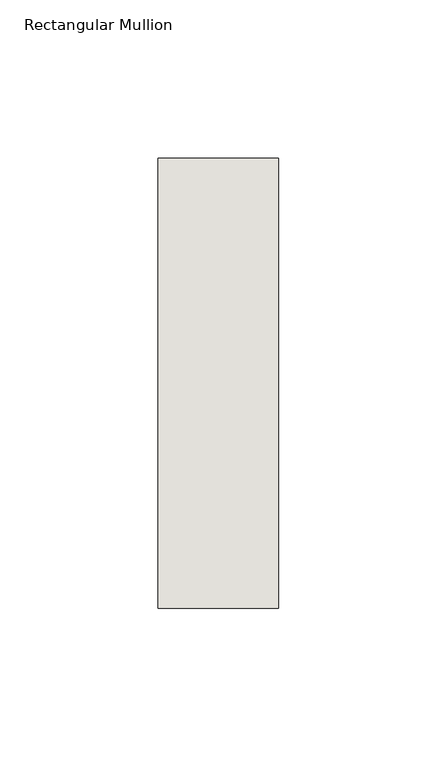
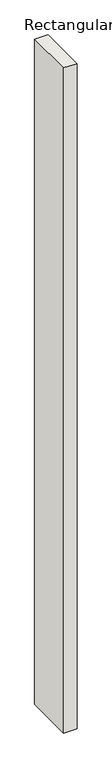
"""IFC4 building model written with IfcOpenShell, lengths in millimetres: wall geometry, Rectangular Mullion : NLRS_21_CWM_hsb-regel 38x142_gen_rsf."""

import ifcopenshell
import ifcopenshell.guid

model = None  # the IFC model being written
_history = None  # IfcOwnerHistory: only IFC2X3 demands one
_inside = {}  # id of a spatial element -> (the spatial element, [elements in it])
_under = {}  # id of a project, library or spatial element -> (it, [spatial elements below it])
_declared = {}  # id of a project -> (the project, [libraries it declares])
_typed = {}  # id of a type object -> (the type object, [elements of that type])
_made_of = {}  # id of a material, layer set ... -> (it, [elements and type objects made of it])


def new_model(schema):
    """Start an empty IFC model of exactly this schema.

    Asked for "IFC4X3", IfcOpenShell would pick the latest addendum, in which some entities
    have other attributes; the version numbers below select the first issue.
    IFC2X3 requires an IfcOwnerHistory on every rooted entity: one is made here for all.
    """
    global model, _history
    if schema == "IFC4X3":
        model = ifcopenshell.file(schema_version=(4, 3, 0, 0))
    else:
        model = ifcopenshell.file(schema=schema)
    _inside.clear()
    _under.clear()
    _declared.clear()
    _typed.clear()
    _made_of.clear()
    _history = None
    if model.schema == "IFC2X3":
        org = make("IfcOrganization", Name="unknown")
        user = make(
            "IfcPersonAndOrganization",
            ThePerson=make("IfcPerson", FamilyName="unknown"),
            TheOrganization=org,
        )
        app = make(
            "IfcApplication",
            ApplicationDeveloper=org,
            Version="unknown",
            ApplicationFullName="unknown",
            ApplicationIdentifier="unknown",
        )
        _history = make(
            "IfcOwnerHistory",
            OwningUser=user,
            OwningApplication=app,
            ChangeAction="ADDED",
            CreationDate=0,
        )
    return model


def make(cls, **values):
    """One entity of the class cls with the attributes given. An attribute that is None is left unset."""
    return model.create_entity(
        cls, **{name: value for name, value in values.items() if value is not None}
    )


def rooted(cls, **values):
    """An entity with a GlobalId (a new one), such as an element, a storey or a relation."""
    return make(cls, GlobalId=ifcopenshell.guid.new(), OwnerHistory=_history, **values)


def si_unit(unit_type, name, prefix=None):
    """IfcSIUnit, for example si_unit("LENGTHUNIT", "METRE", prefix="MILLI")."""
    return make("IfcSIUnit", UnitType=unit_type, Prefix=prefix, Name=name)


def assignment(units):
    """IfcUnitAssignment: the units of a project."""
    return None if units is None else make("IfcUnitAssignment", Units=units)


def point(xyz):
    """IfcCartesianPoint."""
    return None if xyz is None else make("IfcCartesianPoint", Coordinates=xyz)


def direction(xyz):
    """IfcDirection."""
    return None if xyz is None else make("IfcDirection", DirectionRatios=xyz)


def frame(location, z_axis=None, x_axis=None):
    """IfcAxis2Placement3D, a coordinate frame: its origin and axes. An axis left out is left unset."""
    return make(
        "IfcAxis2Placement3D",
        Location=point(location),
        Axis=direction(z_axis),
        RefDirection=direction(x_axis),
    )


def origin():
    """The frame at (0, 0, 0) with its axes left unset."""
    return frame((0.0, 0.0, 0.0))


def place(relative_to, where):
    """IfcLocalPlacement: puts the frame where relative to a parent placement (None: the world)."""
    return make(
        "IfcLocalPlacement", PlacementRelTo=relative_to, RelativePlacement=where
    )


def context(
    kind, dimensions, precision=None, world=None, true_north=None, identifier=None
):
    """IfcGeometricRepresentationContext, for example the 3D "Model" context."""
    return make(
        "IfcGeometricRepresentationContext",
        ContextIdentifier=identifier,
        ContextType=kind,
        CoordinateSpaceDimension=dimensions,
        Precision=precision,
        WorldCoordinateSystem=world,
        TrueNorth=true_north,
    )


def project(units=None, contexts=None):
    """IfcProject with its units and contexts."""
    return rooted(
        "IfcProject",
        Name="project",
        RepresentationContexts=contexts,
        UnitsInContext=assignment(units),
    )


def spatial(cls, under=None, at=None, **own):
    """A site, building, storey or space (cls), placed at a placement, below another one or the project."""
    s = rooted(cls, ObjectPlacement=at, **own)
    if under is not None:
        _under.setdefault(under.id(), (under, []))[1].append(s)
    return s


def polyline(points):
    """IfcPolyline through the points."""
    return make("IfcPolyline", Points=[point(p) for p in points])


def outline(outer, holes=None, kind="AREA"):
    """IfcArbitraryClosedProfileDef: a profile drawn as a closed curve; with holes, ...WithVoids."""
    if holes is None:
        return make("IfcArbitraryClosedProfileDef", ProfileType=kind, OuterCurve=outer)
    return make(
        "IfcArbitraryProfileDefWithVoids",
        ProfileType=kind,
        OuterCurve=outer,
        InnerCurves=holes,
    )


def extrude(swept, where, along, depth):
    """IfcExtrudedAreaSolid: the profile swept, set in the frame where, extruded along a direction by depth."""
    return make(
        "IfcExtrudedAreaSolid",
        SweptArea=swept,
        Position=where,
        ExtrudedDirection=direction(along),
        Depth=depth,
    )


def shape(context_of_items, identifier, shape_type, items):
    """IfcShapeRepresentation: the items that make up one representation, for example the "Body"."""
    return make(
        "IfcShapeRepresentation",
        ContextOfItems=context_of_items,
        RepresentationIdentifier=identifier,
        RepresentationType=shape_type,
        Items=items,
    )


def source(mapping_origin, context_of_items, identifier, shape_type, items):
    """IfcRepresentationMap: a shape defined once, which mapped items show again and again."""
    return make(
        "IfcRepresentationMap",
        MappingOrigin=mapping_origin,
        MappedRepresentation=shape(context_of_items, identifier, shape_type, items),
    )


def transform(
    local_origin,
    x_axis=None,
    y_axis=None,
    z_axis=None,
    scale=None,
    scale2=None,
    scale3=None,
    uniform=True,
):
    """IfcCartesianTransformationOperator3D, or its non-uniform kind. x_axis, y_axis, z_axis: its Axis1, 2, 3."""
    if uniform:
        return make(
            "IfcCartesianTransformationOperator3D",
            Axis1=direction(x_axis),
            Axis2=direction(y_axis),
            LocalOrigin=point(local_origin),
            Scale=scale,
            Axis3=direction(z_axis),
        )
    return make(
        "IfcCartesianTransformationOperator3DnonUniform",
        Axis1=direction(x_axis),
        Axis2=direction(y_axis),
        LocalOrigin=point(local_origin),
        Scale=scale,
        Axis3=direction(z_axis),
        Scale2=scale2,
        Scale3=scale3,
    )


def mapped(mapping_source, mapping_target):
    """IfcMappedItem: shows the shape of a source again, moved by a transform."""
    return make(
        "IfcMappedItem", MappingSource=mapping_source, MappingTarget=mapping_target
    )


def made_of(thing, what):
    """Note that an element or type object is made of a material, layer set ...; save() writes the relation."""
    if what is not None:
        _made_of.setdefault(what.id(), (what, []))[1].append(thing)
    return thing


def element(
    cls,
    number,
    at=None,
    inside=None,
    cuts=None,
    type_object=None,
    material=None,
    context=None,
    identifier="Body",
    shape_type=None,
    held_by="IfcProductDefinitionShape",
    body=None,
    shapes=None,
    **own,
):
    """One element of the class cls, such as IfcWall. Its Tag is "e" and its number.

    at: its placement. inside: the storey or other place that contains it. cuts: it is an
    opening in that element (IfcRelVoidsElement). A single representation is given by context,
    identifier, shape_type and body (its items); several are given by shapes. held_by: the class
    of the entity that holds the representations. save() writes the other relations.
    """
    e = rooted(cls, Tag="e%d" % number, ObjectPlacement=at, **own)
    if body is not None:
        shapes = [shape(context, identifier, shape_type, body)]
    if shapes is not None:
        e.Representation = make(held_by, Representations=shapes)
    if inside is not None:
        _inside.setdefault(inside.id(), (inside, []))[1].append(e)
    if cuts is not None:
        rooted(
            "IfcRelVoidsElement", RelatingBuildingElement=cuts, RelatedOpeningElement=e
        )
    if type_object is not None:
        _typed.setdefault(type_object.id(), (type_object, []))[1].append(e)
    return made_of(e, material)


def aggregate(whole, parts):
    """IfcRelAggregates: a whole, such as a stair, and the parts it consists of."""
    return rooted("IfcRelAggregates", RelatingObject=whole, RelatedObjects=parts)


def save(model, path):
    """Write the relations noted so far, then the file.

    IfcRelAggregates (storeys below a building ...), IfcRelContainedInSpatialStructure (elements
    in a storey), IfcRelDefinesByType, IfcRelAssociatesMaterial and IfcRelDeclares: one each for
    every whole, place, type object, material and project.
    """
    for whole, parts in _under.values():
        aggregate(whole, parts)
    for where, things in _inside.values():
        rooted(
            "IfcRelContainedInSpatialStructure",
            RelatedElements=things,
            RelatingStructure=where,
        )
    for kind, things in _typed.values():
        rooted("IfcRelDefinesByType", RelatedObjects=things, RelatingType=kind)
    for what, things in _made_of.values():
        rooted("IfcRelAssociatesMaterial", RelatedObjects=things, RelatingMaterial=what)
    for by, libraries in _declared.values():
        rooted("IfcRelDeclares", RelatingContext=by, RelatedDefinitions=libraries)
    model.write(path)


def rectangular_mullion_39ed0f6f(model_context):
    return source(origin(), model_context, "Body", "SweptSolid", [
        extrude(outline(polyline([(-38.0, -71.0), (-38.0, 71.0), (0.0, 71.0), (0.0, -71.0), (-38.0, -71.0)])), frame((0.0, 0.0, -2000.0), z_axis=(0.0, 0.0, 1.0), x_axis=(1.0, 0.0, 0.0)), (0.0, 0.0, 1.0), 2000.0),
    ])


if __name__ == "__main__":
    model = new_model("IFC4")
    model_context = context("Model", 3, world=origin())
    ifc_project = project(units=[si_unit("LENGTHUNIT", "METRE", prefix="MILLI")], contexts=[model_context])
    site = spatial("IfcSite", under=ifc_project)
    building = spatial("IfcBuilding", under=site)
    placement = place(None, origin())
    rectangular_mullion_shape = rectangular_mullion_39ed0f6f(model_context)
    element("IfcWall", 1, ObjectType="Rectangular Mullion : NLRS_21_CWM_hsb-regel 38x142_gen_rsf", at=placement, inside=building, context=model_context, shape_type="MappedRepresentation", body=[
        mapped(rectangular_mullion_shape, transform((0.0, 0.0, 0.0), x_axis=(1.0, 0.0, 0.0), y_axis=(0.0, 1.0, 0.0), z_axis=(0.0, 0.0, 1.0))),
    ])
    save(model, "model.ifc")

# Revit data of these elements
# Type "Rectangular Mullion : NLRS_21_CWM_hsb-regel 38x142_gen_rsf"
#   Type IfcGUID = "07M7mRoiH1CR8m_RSKIwpF"
#   Assembly Code = "21.10"
#   IfcExportAs = "IfcWall"
#   built-in parameter 1007322 = 0.465879 (stored number, unit not read)
#   built-in parameter 1007321 = 0.062336 (stored number, unit not read)
#   built-in parameter 1007320 = 0.062336 (stored number, unit not read)
# Element 1 (IfcWall, "Rectangular Mullion : NLRS_21_CWM_hsb-regel 38x142_gen_rsf")
#   Materials on its faces: "NLRS_i2_hout naaldhout vuren_gen_rsf"
# Materials
#   "NLRS_i2_hout naaldhout vuren_gen_rsf": class "I - Hout", colour RGB 234 199 147, transparency 0, Keynote = "i2", Manufacturer = "Revit Standards Foundation", URL = "www.revitstandards.org", Description = "hout vuren", Cost = 0
